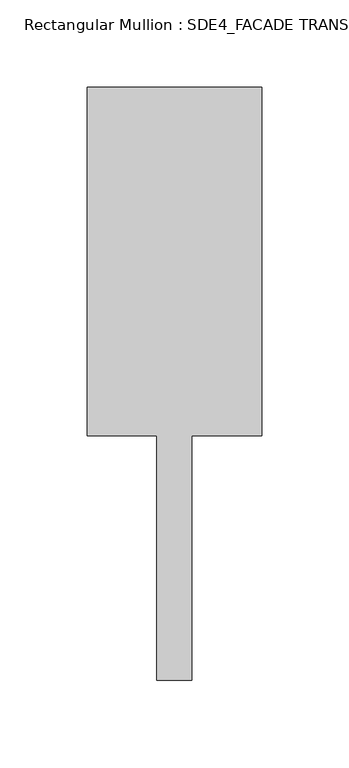
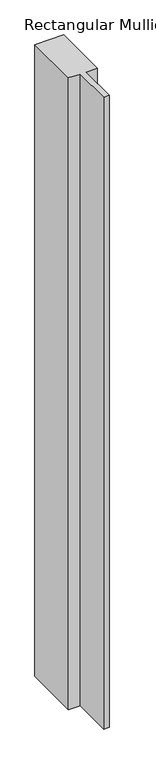
"""IFC4 building model written with IfcOpenShell, lengths in millimetres: member geometry, Rectangular Mullion : SDE4_FACADE TRANSOM TYPE 1."""

from ifc_helpers import new_model, si_unit, frame, origin, place, context, project, spatial, polyline, outline, extrude, source, transform, mapped, element, save


def rectangular_mullion_sde4_facade_transom_type_1_648ba6ff(model_context):
    return source(origin(), model_context, "Body", "SweptSolid", [
        extrude(outline(polyline([(50.0, 132.5), (50.0, -67.5), (10.0, -67.5), (10.0, -207.5), (-10.0, -207.5), (-10.0, -67.5), (-50.0, -67.5), (-50.0, 132.5), (50.0, 132.5)])), frame((0.0, 0.0, -2300.0), z_axis=(0.0, 0.0, 1.0), x_axis=(1.0, 0.0, 0.0)), (0.0, 0.0, 1.0), 2300.0),
    ])


if __name__ == "__main__":
    model = new_model("IFC4")
    model_context = context("Model", 3, world=origin())
    ifc_project = project(units=[si_unit("LENGTHUNIT", "METRE", prefix="MILLI")], contexts=[model_context])
    site = spatial("IfcSite", under=ifc_project)
    building = spatial("IfcBuilding", under=site)
    placement = place(None, origin())
    rectangular_mullion_sde4_facade_transom_type_1_shape = rectangular_mullion_sde4_facade_transom_type_1_648ba6ff(model_context)
    element("IfcMember", 1, ObjectType="Rectangular Mullion : SDE4_FACADE TRANSOM TYPE 1", at=placement, inside=building, context=model_context, shape_type="MappedRepresentation", body=[
        mapped(rectangular_mullion_sde4_facade_transom_type_1_shape, transform((0.0, 0.0, 0.0), x_axis=(1.0, 0.0, 0.0), y_axis=(0.0, 1.0, 0.0), z_axis=(0.0, 0.0, 1.0))),
    ])
    save(model, "model.ifc")

# Revit data of these elements
# Type "Rectangular Mullion : SDE4_FACADE TRANSOM TYPE 1"
#   built-in parameter 1007322 = 1.11549 (stored number, unit not read)
#   built-in parameter 1007321 = 0.164042 (stored number, unit not read)
#   built-in parameter 1007320 = 0.164042 (stored number, unit not read)
